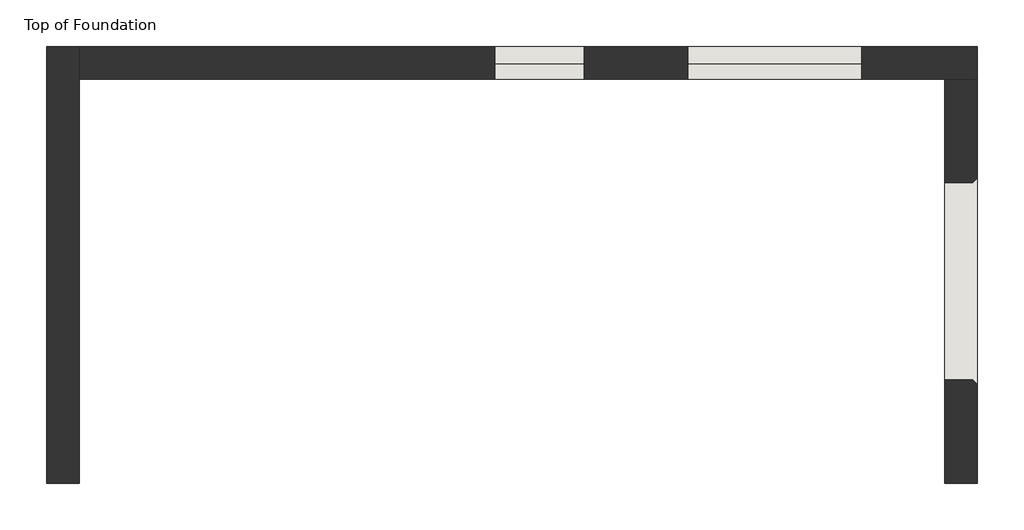
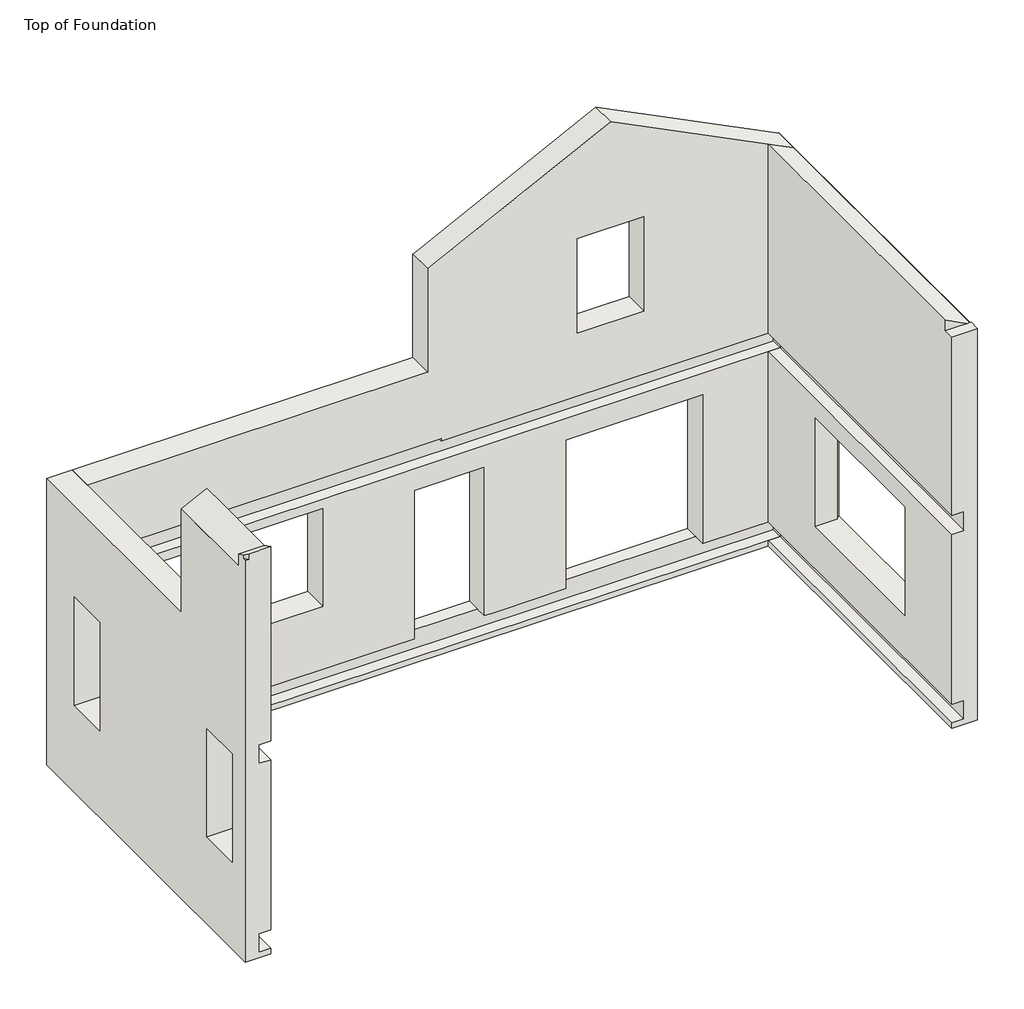
# One storey: 3 walls.
"""IFC4 building model written with IfcOpenShell, lengths in millimetres."""

from ifc_helpers import new_model, si_unit, origin, place, context, project, spatial, faceted_brep, element, save

model = new_model("IFC4")

# Units and contexts
model_context = context("Model", 3, world=origin())
ifc_project = project(units=[si_unit("LENGTHUNIT", "METRE", prefix="MILLI")], contexts=[model_context])

# Site, building, storey
site = spatial("IfcSite", under=ifc_project)
building = spatial("IfcBuilding", under=site)
storey = spatial("IfcBuildingStorey", under=building, Name="Top of Foundation", Elevation=-349.25)

# Walls
placement = place(None, origin())
element("IfcWall", 1, ObjectType="Exterior - Brick on Mtl. Stud", at=placement, inside=storey, context=model_context, shape_type="Brep", body=[
    faceted_brep([(-5636.7553068, 3152.0888758, -349.25), (-5636.7553068, 7524.0638758, -349.25), (-5636.7553068, 7876.4888758, -349.25), (-5636.7553068, 7876.4888758, 3810.0), (-5636.7553068, 7524.0638758, 3810.0), (-5636.7553068, 4676.0888758, 3810.0), (-5636.7553068, 4676.0888758, 5486.4), (-5636.7553068, 4323.6638758, 5486.4), (-5636.7553068, 3304.4888758, 5486.4), (-5636.7553068, 3304.4888758, 5488.5342644), (-5636.7553068, 3152.0888758, 5564.7342644), (-5636.7553068, 3152.0888758, 2743.2), (-5636.7553068, 4323.6638758, 2743.2), (-5636.7553068, 4488.7638758, 2743.2), (-5636.7553068, 4488.7638758, 2781.3), (-5636.7553068, 4676.0888758, 2781.3), (-5636.7553068, 7524.0638758, 2781.3), (-5636.7553068, 7689.1638758, 2781.3), (-5636.7553068, 7689.1638758, 2470.15), (-5636.7553068, 7524.0638758, 2470.15), (-5636.7553068, 7219.2638758, 2470.15), (-5636.7553068, 7219.2638758, 914.4), (-5636.7553068, 6609.6638758, 914.4), (-5636.7553068, 6609.6638758, 2470.15), (-5636.7553068, 4066.4888758, 2470.15), (-5636.7553068, 4066.4888758, 914.4), (-5636.7553068, 3456.8888758, 914.4), (-5636.7553068, 3456.8888758, 2470.15), (-5636.7553068, 3152.0888758, 2470.15), (-5636.7553068, 3152.0888758, 0.0), (-5636.7553068, 7524.0638758, 0.0), (-5636.7553068, 7689.1638758, 0.0), (-5636.7553068, 7689.1638758, -273.05), (-5636.7553068, 7524.0638758, -273.05), (-5636.7553068, 3152.0888758, -273.05), (-5989.1803068, 7876.4888758, -349.25), (-5989.1803068, 3152.0888758, -349.25), (-5989.1803068, 3152.0888758, 5486.4), (-5989.1803068, 3199.7138758, 5486.4), (-5989.1803068, 3199.7138758, 5540.9217644), (-5989.1803068, 3304.4888758, 5488.5342644), (-5989.1803068, 3304.4888758, 5312.3217644), (-5989.1803068, 4676.0888758, 5312.3217644), (-5989.1803068, 4676.0888758, 3810.0), (-5989.1803068, 7876.4888758, 3810.0), (-5989.1803068, 3456.8888758, 2489.2), (-5989.1803068, 3456.8888758, 914.4), (-5989.1803068, 4066.4888758, 914.4), (-5989.1803068, 4066.4888758, 2489.2), (-5989.1803068, 6609.6638758, 2489.2), (-5989.1803068, 6609.6638758, 914.4), (-5989.1803068, 7219.2638758, 914.4), (-5989.1803068, 7219.2638758, 2489.2), (-5801.8553068, 3152.0888758, -273.05), (-5801.8553068, 3152.0888758, 0.0), (-5801.8553068, 3152.0888758, 2470.15), (-5801.8553068, 3152.0888758, 2743.2), (-5941.5553068, 3152.0888758, 5564.7342644), (-5941.5553068, 3152.0888758, 5486.4), (-5984.911778, 4676.0888758, 5312.3217644), (-5937.286778, 3304.4888758, 5336.1342644), (-5984.911778, 3304.4888758, 5312.3217644), (-5801.8553068, 3456.8888758, 2489.2), (-5801.8553068, 3456.8888758, 2470.15), (-5801.8553068, 4066.4888758, 2470.15), (-5801.8553068, 4066.4888758, 2489.2), (-5801.8553068, 6609.6638758, 2489.2), (-5801.8553068, 6609.6638758, 2470.15), (-5801.8553068, 7219.2638758, 2470.15), (-5801.8553068, 7219.2638758, 2489.2), (-5801.8553068, 7689.1638758, -273.05), (-5801.8553068, 7689.1638758, 0.0), (-5801.8553068, 7689.1638758, 2470.15), (-5801.8553068, 4488.7638758, 2470.15), (-5801.8553068, 4488.7638758, 2743.2), (-5801.8553068, 7689.1638758, 2781.3), (-5801.8553068, 4488.7638758, 2781.3)], [[[0, 1, 2, 3, 4, 5, 6, 7, 8, 9, 10, 11, 12, 13, 14, 15, 16, 17, 18, 19, 20, 21, 22, 23, 24, 25, 26, 27, 28, 29, 30, 31, 32, 33, 34]], [[35, 36, 37, 38, 39, 40, 41, 42, 43, 44], [45, 46, 47, 48], [49, 50, 51, 52]], [[3, 2, 35, 44]], [[2, 1, 0, 36, 35]], [[37, 36, 0, 34, 53, 54, 29, 28, 55, 56, 11, 10, 57, 58]], [[5, 4, 3, 44, 43]], [[6, 5, 43, 42, 59]], [[41, 40, 9, 8, 60, 61]], [[38, 37, 58]], [[38, 58, 57, 39]], [[8, 7, 6, 59, 61, 60]], [[42, 41, 61, 59]], [[10, 9, 40, 39, 57]], [[46, 45, 62, 63, 27, 26]], [[47, 46, 26, 25]], [[48, 47, 25, 24, 64, 65]], [[45, 48, 65, 62]], [[50, 49, 66, 67, 23, 22]], [[51, 50, 22, 21]], [[52, 51, 21, 20, 68, 69]], [[49, 52, 69, 66]], [[70, 53, 34, 33, 32]], [[71, 31, 30, 29, 54]], [[71, 70, 32, 31]], [[70, 71, 54, 53]], [[72, 68, 20, 19, 18]], [[64, 24, 23, 67, 73]], [[63, 55, 28, 27]], [[56, 74, 13, 12, 11]], [[55, 63, 62, 65, 64, 73, 67, 66, 69, 68, 72, 75, 76, 74, 56]], [[76, 75, 17, 16, 15, 14]], [[75, 72, 18, 17]], [[74, 76, 14, 13]]]),
])
element("IfcWall", 2, ObjectType="Exterior - Brick on Mtl. Stud", at=placement, inside=storey, context=model_context, shape_type="Brep", body=[
    faceted_brep([(-5636.7553068, 7524.0638758, -349.25), (3716.7946932, 7524.0638758, -349.25), (4069.2196932, 7524.0638758, -349.25), (4069.2196932, 7524.0638758, 5312.3217644), (4064.9511643, 7524.0638758, 5312.3217644), (3716.7946932, 7524.0638758, 5486.4), (1554.6196932, 7524.0638758, 6567.4875), (-607.5553068, 7524.0638758, 5486.4), (-955.711778, 7524.0638758, 5312.3217644), (-959.9803068, 7524.0638758, 5312.3217644), (-959.9803068, 7524.0638758, 3810.0), (-5636.7553068, 7524.0638758, 3810.0), (-5636.7553068, 7524.0638758, 2781.3), (-772.6553068, 7524.0638758, 2781.3), (-772.6553068, 7524.0638758, 2743.2), (-607.5553068, 7524.0638758, 2743.2), (3881.8946932, 7524.0638758, 2743.2), (3881.8946932, 7524.0638758, 2470.15), (43.3196932, 7524.0638758, 2470.15), (-77.3303068, 7524.0638758, 2470.15), (-1480.6803068, 7524.0638758, 2470.15), (-1601.3303068, 7524.0638758, 2470.15), (-5636.7553068, 7524.0638758, 2470.15), (-5636.7553068, 7524.0638758, 0.0), (-1601.3303068, 7524.0638758, 0.0), (-1480.6803068, 7524.0638758, 0.0), (-1144.1303068, 7524.0638758, 0.0), (-1144.1303068, 7524.0638758, 2159.0), (-178.9303068, 7524.0638758, 2159.0), (-178.9303068, 7524.0638758, 0.0), (-77.3303068, 7524.0638758, 0.0), (43.3196932, 7524.0638758, 0.0), (940.2571932, 7524.0638758, 0.0), (940.2571932, 7524.0638758, 2159.0), (2819.8571932, 7524.0638758, 2159.0), (2819.8571932, 7524.0638758, 0.0), (3881.8946932, 7524.0638758, 0.0), (3881.8946932, 7524.0638758, -273.05), (-5636.7553068, 7524.0638758, -273.05), (1097.4196932, 7524.0638758, 3657.6), (1097.4196932, 7524.0638758, 5029.2), (2011.8196932, 7524.0638758, 5029.2), (2011.8196932, 7524.0638758, 3657.6), (-2399.8428068, 7524.0638758, 2336.8), (-2399.8428068, 7524.0638758, 914.4), (-4838.2428068, 7524.0638758, 914.4), (-4838.2428068, 7524.0638758, 2336.8), (4069.2196932, 7876.4888758, -349.25), (-5636.7553068, 7876.4888758, -349.25), (-5636.7553068, 7876.4888758, 3810.0), (-959.9803068, 7876.4888758, 3810.0), (-959.9803068, 7876.4888758, 5312.3217644), (-955.711778, 7876.4888758, 5312.3217644), (1554.6196932, 7876.4888758, 6567.4875), (4064.9511643, 7876.4888758, 5312.3217644), (4069.2196932, 7876.4888758, 5312.3217644), (1097.4196932, 7876.4888758, 5029.2), (1097.4196932, 7876.4888758, 3657.6), (2011.8196932, 7876.4888758, 3657.6), (2011.8196932, 7876.4888758, 5029.2), (-1144.1303068, 7876.4888758, 2159.0), (-1144.1303068, 7876.4888758, 0.0), (-178.9303068, 7876.4888758, 0.0), (-178.9303068, 7876.4888758, 2159.0), (-2399.8428068, 7876.4888758, 914.4), (-2399.8428068, 7876.4888758, 2336.8), (-4838.2428068, 7876.4888758, 2336.8), (-4838.2428068, 7876.4888758, 914.4), (2819.8571932, 7876.4888758, 0.0), (2819.8571932, 7876.4888758, 2159.0), (940.2571932, 7876.4888758, 2159.0), (940.2571932, 7876.4888758, 0.0), (-5636.7553068, 7689.1638758, -273.05), (-5636.7553068, 7689.1638758, 0.0), (-5636.7553068, 7689.1638758, 2470.15), (-5636.7553068, 7689.1638758, 2781.3), (4069.2196932, 7571.6888758, -349.25), (-1144.1303068, 7689.1638758, 0.0), (-178.9303068, 7689.1638758, 0.0), (2819.8571932, 7689.1638758, 0.0), (940.2571932, 7689.1638758, 0.0), (3881.8946932, 7689.1638758, -273.05), (3881.8946932, 7689.1638758, 0.0), (3881.8946932, 7689.1638758, 2470.15), (-772.6553068, 7689.1638758, 2470.15), (-772.6553068, 7689.1638758, 2743.2), (3881.8946932, 7689.1638758, 2743.2), (-772.6553068, 7689.1638758, 2781.3)], [[[0, 1, 2, 3, 4, 5, 6, 7, 8, 9, 10, 11, 12, 13, 14, 15, 16, 17, 18, 19, 20, 21, 22, 23, 24, 25, 26, 27, 28, 29, 30, 31, 32, 33, 34, 35, 36, 37, 38], [39, 40, 41, 42], [43, 44, 45, 46]], [[47, 48, 49, 50, 51, 52, 53, 54, 55], [56, 57, 58, 59], [60, 61, 62, 63], [64, 65, 66, 67], [68, 69, 70, 71]], [[49, 48, 0, 38, 72, 73, 23, 22, 74, 75, 12, 11]], [[3, 2, 76, 47, 55]], [[2, 1, 0, 48, 47, 76]], [[11, 10, 50, 49]], [[10, 9, 51, 50]], [[51, 9, 8, 52]], [[8, 7, 6, 53, 52]], [[6, 5, 4, 54, 53]], [[3, 55, 54, 4]], [[57, 56, 40, 39]], [[58, 57, 39, 42]], [[59, 58, 42, 41]], [[56, 59, 41, 40]], [[27, 26, 77, 61, 60]], [[28, 27, 60, 63]], [[29, 28, 63, 62, 78]], [[62, 61, 77, 78]], [[44, 64, 67, 45]], [[65, 43, 46, 66]], [[64, 44, 43, 65]], [[66, 46, 45, 67]], [[69, 68, 79, 35, 34]], [[70, 69, 34, 33]], [[71, 70, 33, 32, 80]], [[68, 71, 80, 79]], [[37, 81, 72, 38]], [[79, 82, 36, 35]], [[78, 80, 32, 31, 30, 29]], [[73, 77, 26, 25, 24, 23]], [[81, 82, 79, 80, 78, 77, 73, 72]], [[82, 81, 37, 36]], [[74, 22, 21, 20, 19, 18, 17, 83, 84]], [[85, 86, 16, 15, 14]], [[74, 84, 83, 86, 85, 87, 75]], [[86, 83, 17, 16]], [[75, 87, 13, 12]], [[87, 85, 14, 13]]]),
])
element("IfcWall", 3, ObjectType="Exterior - Brick on Mtl. Stud", at=placement, inside=storey, context=model_context, shape_type="Brep", body=[
    faceted_brep([(3716.7946932, 7524.0638758, -349.25), (3716.7946932, 3152.0888758, -349.25), (3716.7946932, 3152.0888758, -273.05), (3716.7946932, 7524.0638758, -273.05), (3716.7946932, 3304.4888758, 5336.1342644), (3716.7946932, 3304.4888758, 5486.4), (3716.7946932, 3844.2388758, 5486.4), (3716.7946932, 3964.8888758, 5486.4), (3716.7946932, 7524.0638758, 5486.4), (3716.7946932, 7524.0638758, 2743.2), (3716.7946932, 3964.8888758, 2743.2), (3716.7946932, 3844.2388758, 2743.2), (3716.7946932, 3152.0888758, 2743.2), (3716.7946932, 3152.0888758, 5336.1342644), (3716.7946932, 7524.0638758, 0.0), (3716.7946932, 3152.0888758, 0.0), (3716.7946932, 3152.0888758, 2470.15), (3716.7946932, 7524.0638758, 2470.15), (3716.7946932, 6404.8763758, 2184.4), (3716.7946932, 4271.2763758, 2184.4), (3716.7946932, 4271.2763758, 609.6), (3716.7946932, 6404.8763758, 609.6), (4069.2196932, 3152.0888758, -349.25), (4069.2196932, 7524.0638758, -349.25), (4069.2196932, 7524.0638758, 5312.3217644), (4069.2196932, 3304.4888758, 5312.3217644), (4069.2196932, 3304.4888758, 5336.1342644), (4069.2196932, 3152.0888758, 5336.1342644), (4069.2196932, 4221.8849671, 2184.4), (4069.2196932, 6454.2677845, 2184.4), (4069.2196932, 6454.2677845, 609.6), (4069.2196932, 4221.8849671, 609.6), (3881.8946932, 3152.0888758, 2743.2), (3881.8946932, 3152.0888758, 2470.15), (3881.8946932, 3152.0888758, 0.0), (3881.8946932, 3152.0888758, -273.05), (3881.8946932, 7524.0638758, -273.05), (3881.8946932, 7524.0638758, 0.0), (3881.8946932, 7524.0638758, 2470.15), (3881.8946932, 7524.0638758, 2743.2), (4064.9511643, 7524.0638758, 5312.3217644), (4064.9511643, 3304.4888758, 5312.3217644), (4017.3261643, 3304.4888758, 5336.1342644), (4019.8282845, 6404.8763758, 2184.4), (4019.8282845, 4271.2763758, 2184.4), (4019.8282845, 6404.8763758, 609.6), (4019.8282845, 4271.2763758, 609.6)], [[[0, 1, 2, 3]], [[4, 5, 6, 7, 8, 9, 10, 11, 12, 13]], [[14, 15, 16, 17], [18, 19, 20, 21]], [[22, 23, 24, 25, 26, 27], [28, 29, 30, 31]], [[1, 0, 23, 22]], [[22, 27, 13, 12, 32, 33, 16, 15, 34, 35, 2, 1]], [[24, 23, 0, 3, 36, 37, 14, 17, 38, 39, 9, 8, 40]], [[26, 25, 41, 42]], [[4, 13, 27, 26, 42]], [[8, 7, 6, 5, 42, 41, 40]], [[25, 24, 40, 41]], [[5, 4, 42]], [[43, 29, 28, 44, 19, 18]], [[45, 21, 20, 46, 31, 30]], [[43, 18, 21, 45]], [[19, 44, 46, 20]], [[44, 28, 31, 46]], [[29, 43, 45, 30]], [[35, 36, 3, 2]], [[37, 34, 15, 14]], [[36, 35, 34, 37]], [[33, 38, 17, 16]], [[39, 32, 12, 11, 10, 9]], [[38, 33, 32, 39]]]),
])

save(model, "model.ifc")

# Revit data of these elements
# Type "Exterior - Brick on Mtl. Stud"
#   Assembly Code = "B2010158"
#   Layers, outside or top first: 0' - 3 5/8" "Brick, Common" (function 4); 0' - 3" "Air" (function 3); 0' - 0" "Air Infiltration Barrier" (function 100); 0' - 0 3/4" "Plywood, Sheathing" (function 2); 0' - 6" "Metal Stud Layer" (function 1); 0' - 0" "Vapor Retarder" (function 100); 0' - 0 1/2" "Gypsum Wall Board" (function 5)
# Elements 1, 2 (IfcWall, "Exterior - Brick on Mtl. Stud")
#   Top Offset = 0' - 0"
#   Base Offset = 0' - 0"
#   wall height = 19' - 1 3/4"
#   Phase Created = New Construction
#   Base Constraint = Top of Foundation
#   Top Constraint = Roof
#   Materials on its faces: "Default Wall", "Brick, Common", "Gypsum Wall Board"
# Element 3 (IfcWall, "Exterior - Brick on Mtl. Stud")
#   Top Offset = 0' - 0"
#   Base Offset = 0' - 0"
#   wall height = 19' - 1 3/4"
#   Phase Created = New Construction
#   Base Constraint = Top of Foundation
#   Top Constraint = Roof
#   Materials on its faces: "Default Wall", "Gypsum Wall Board", "Brick, Common"
# Materials
#   "Brick, Common": class "Masonry", colour RGB 170 98 104, transparency 0, Description = "Common brick", Cost = 0
#   "Air": class "Gas", colour RGB 255 255 255, transparency 0, Description = "Air", Cost = 0
#   "Air Infiltration Barrier": class "Generic", colour RGB 127 127 127, transparency 0, Description = "physical material", Cost = 0
#   "Plywood, Sheathing": class "Wood", colour RGB 193 140 64, transparency 0, Description = "Plywood, sheathing grade", Cost = 0
#   "Metal Stud Layer": class "Metal", colour RGB 199 199 199, transparency 0, Description = "Light gauge steel framing, thermal air layer", Cost = 0
#   "Vapor Retarder": class "Generic", colour RGB 127 127 127, transparency 0, Description = "Polyethylene film membrane", Cost = 0
#   "Gypsum Wall Board": class "Generic", colour RGB 127 127 127, transparency 0, Description = "Gypsum Wall Board", Cost = 0
#   "Default Wall": class "Miscellaneous", colour RGB 128 128 128, transparency 0, Cost = 0
